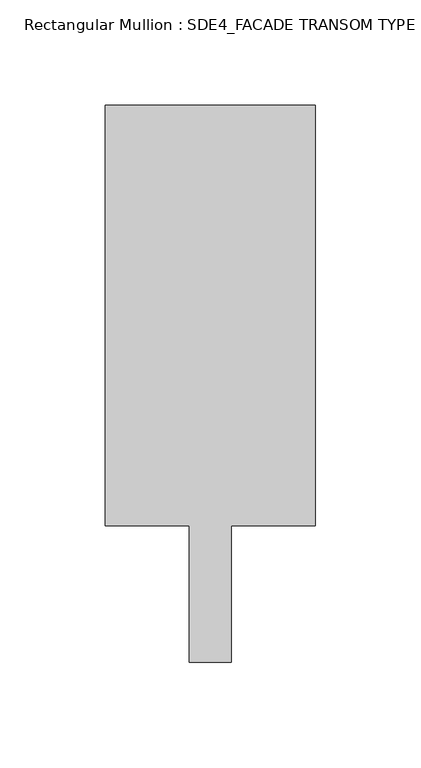
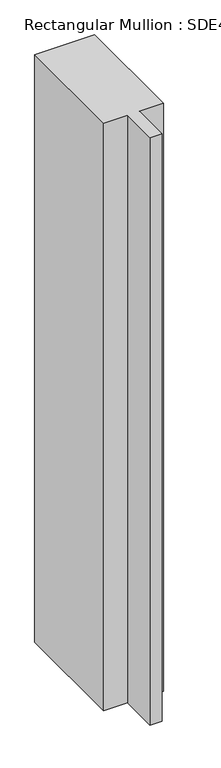
"""IFC4 building model written with IfcOpenShell, lengths in millimetres: member geometry, Rectangular Mullion : SDE4_FACADE TRANSOM TYPE 2."""

from ifc_helpers import new_model, si_unit, frame, origin, place, context, project, spatial, polyline, outline, extrude, source, transform, mapped, element, save


def rectangular_mullion_sde4_facade_transom_type_2_c713611f(model_context):
    return source(origin(), model_context, "Body", "SweptSolid", [
        extrude(outline(polyline([(50.0, 132.5), (50.0, -67.5), (10.0, -67.5), (10.0, -132.5), (-10.0, -132.5), (-10.0, -67.5), (-50.0, -67.5), (-50.0, 132.5), (50.0, 132.5)])), frame((0.0, 0.0, -1039.0), z_axis=(0.0, 0.0, 1.0), x_axis=(1.0, 0.0, 0.0)), (0.0, 0.0, 1.0), 1039.0),
    ])


if __name__ == "__main__":
    model = new_model("IFC4")
    model_context = context("Model", 3, world=origin())
    ifc_project = project(units=[si_unit("LENGTHUNIT", "METRE", prefix="MILLI")], contexts=[model_context])
    site = spatial("IfcSite", under=ifc_project)
    building = spatial("IfcBuilding", under=site)
    placement = place(None, origin())
    rectangular_mullion_sde4_facade_transom_type_2_shape = rectangular_mullion_sde4_facade_transom_type_2_c713611f(model_context)
    element("IfcMember", 1, ObjectType="Rectangular Mullion : SDE4_FACADE TRANSOM TYPE 2", at=placement, inside=building, context=model_context, shape_type="MappedRepresentation", body=[
        mapped(rectangular_mullion_sde4_facade_transom_type_2_shape, transform((0.0, 0.0, 0.0), x_axis=(1.0, 0.0, 0.0), y_axis=(0.0, 1.0, 0.0), z_axis=(0.0, 0.0, 1.0))),
    ])
    save(model, "model.ifc")

# Revit data of these elements
# Type "Rectangular Mullion : SDE4_FACADE TRANSOM TYPE 2"
#   built-in parameter 1007322 = 0.869423 (stored number, unit not read)
#   built-in parameter 1007321 = 0.164042 (stored number, unit not read)
#   built-in parameter 1007320 = 0.164042 (stored number, unit not read)
